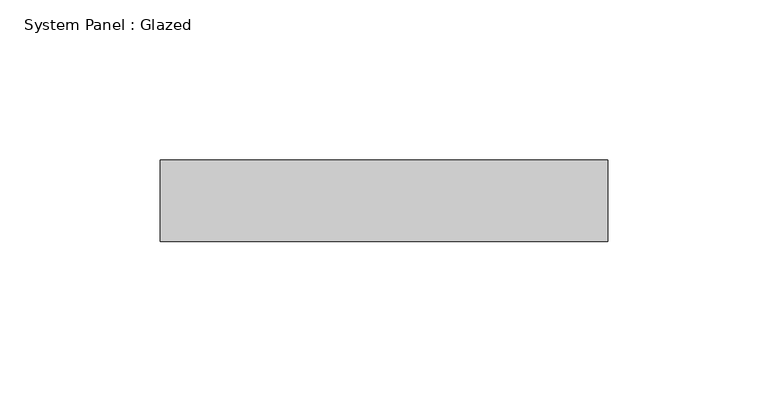
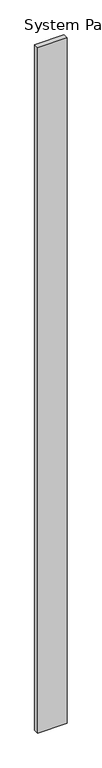
"""IFC4 building model written with IfcOpenShell, lengths in millimetres: plate geometry, System Panel : Glazed."""

from ifc_helpers import new_model, si_unit, origin, origin_with_axes, place, context, project, spatial, polyline, outline, extrude, source, transform, mapped, element, save


def system_panel_glazed_c127a6e8(model_context):
    return source(origin(), model_context, "Body", "SweptSolid", [
        extrude(outline(polyline([(69.649919, 19.05), (-69.649919, 19.05), (-69.649919, 44.45), (69.649919, 44.45), (69.649919, 19.05)])), origin_with_axes(), (0.0, 0.0, 1.0), 3454.4),
    ])


if __name__ == "__main__":
    model = new_model("IFC4")
    model_context = context("Model", 3, world=origin())
    ifc_project = project(units=[si_unit("LENGTHUNIT", "METRE", prefix="MILLI")], contexts=[model_context])
    site = spatial("IfcSite", under=ifc_project)
    building = spatial("IfcBuilding", under=site)
    placement = place(None, origin())
    system_panel_glazed_shape = system_panel_glazed_c127a6e8(model_context)
    element("IfcPlate", 1, ObjectType="System Panel : Glazed", at=placement, inside=building, context=model_context, shape_type="MappedRepresentation", body=[
        mapped(system_panel_glazed_shape, transform((0.0, 0.0, 0.0), x_axis=(1.0, 0.0, 0.0), y_axis=(0.0, 1.0, 0.0), z_axis=(0.0, 0.0, 1.0))),
    ])
    save(model, "model.ifc")

# Revit data of these elements
# Type "System Panel : Glazed"
#   Construction Type Id = "GSP4R"
#   Analytic Construction = "1/8 in Pilkington single glazing"
#   Visual Light Transmittance = 0.9
#   Solar Heat Gain Coefficient = 0.86
#   Heat Transfer Coefficient (U) = 1.18115 BTU/(h·ft²·°F)
#   Define Thermal Properties by = 1
# Element 1 (IfcPlate, "System Panel : Glazed")
#   Materials on its faces: "Glass"
# Materials
#   "Glass": class "Glass", colour RGB 0 128 192, transparency 0.75, Description = "Soda Lime Glass", Cost = 0
